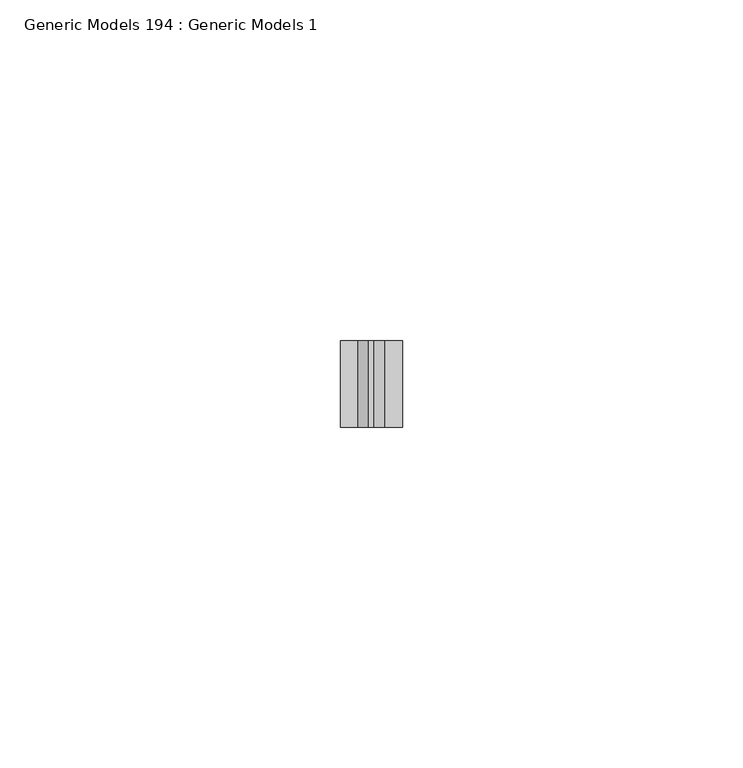
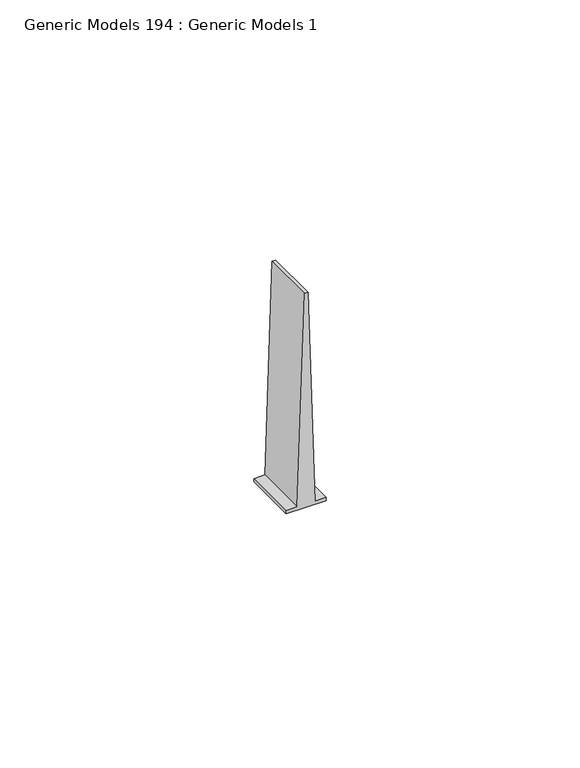
"""IFC4 building model written with IfcOpenShell, lengths in millimetres: proxy geometry, Generic Models 194 : Generic Models 1."""

from ifc_helpers import new_model, si_unit, frame, origin, place, context, project, spatial, polyline, outline, extrude, source, transform, mapped, element, save


def generic_models_194_generic_models_1_857d0d71(model_context):
    return source(origin(), model_context, "Body", "SweptSolid", [
        extrude(outline(polyline([(530.6214294, 52599.8605108), (530.6214294, 52608.9537108), (531.4151794, 52608.9537108), (531.4151794, 52606.4038472), (582.2151794, 52604.8064581), (582.2151794, 52604.0077635), (531.4151794, 52602.4103744), (531.4151794, 52599.8605108), (530.6214294, 52599.8605108)])), frame((0.0, 565.15, 0.0), z_axis=(0.0, 1.0, 0.0), x_axis=(0.0, 0.0, 1.0)), (0.0, 0.0, 1.0), 12.7),
    ])


if __name__ == "__main__":
    model = new_model("IFC4")
    model_context = context("Model", 3, world=origin())
    ifc_project = project(units=[si_unit("LENGTHUNIT", "METRE", prefix="MILLI")], contexts=[model_context])
    site = spatial("IfcSite", under=ifc_project)
    building = spatial("IfcBuilding", under=site)
    placement = place(None, origin())
    generic_models_194_generic_models_1_shape = generic_models_194_generic_models_1_857d0d71(model_context)
    element("IfcBuildingElementProxy", 1, Name="Generic Models 194 : Generic Models 1", ObjectType="Generic Models 194 : Generic Models 1", at=placement, inside=building, context=model_context, shape_type="MappedRepresentation", body=[
        mapped(generic_models_194_generic_models_1_shape, transform((0.0, 0.0, 0.0), x_axis=(1.0, 0.0, 0.0), y_axis=(0.0, 1.0, 0.0), z_axis=(0.0, 0.0, 1.0))),
    ])
    save(model, "model.ifc")

# Revit data of these elements
# Element 1 (IfcBuildingElementProxy, "Generic Models 194 : Generic Models 1")
#   Materials on its faces: "METAL RUNNER CHANNEL; FASTEN @ 24\" O.C."
# Materials
#   "METAL RUNNER CHANNEL; FASTEN @ 24\" O.C.": class "Unassigned", colour RGB 210 209 208, transparency 0, Keynote = "M05121300.02", Cost = 0
